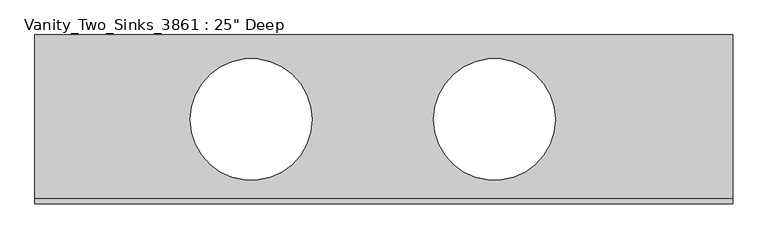
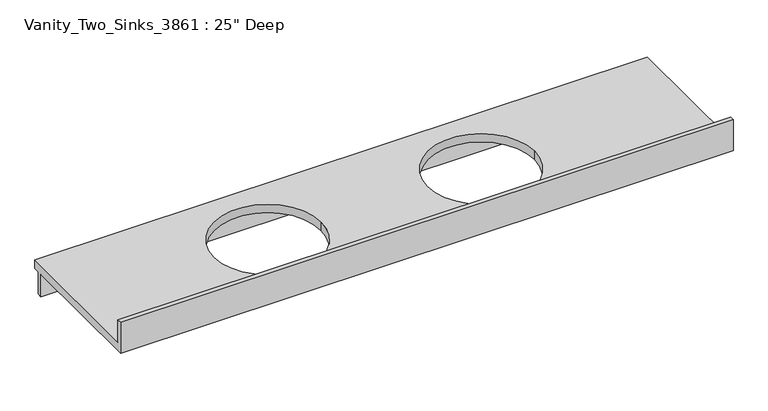
"""IFC4 building model written with IfcOpenShell, lengths in millimetres: furniture geometry."""

import ifcopenshell
import ifcopenshell.guid

model = None  # the IFC model being written
_history = None  # IfcOwnerHistory: only IFC2X3 demands one
_inside = {}  # id of a spatial element -> (the spatial element, [elements in it])
_under = {}  # id of a project, library or spatial element -> (it, [spatial elements below it])
_declared = {}  # id of a project -> (the project, [libraries it declares])
_typed = {}  # id of a type object -> (the type object, [elements of that type])
_made_of = {}  # id of a material, layer set ... -> (it, [elements and type objects made of it])


def new_model(schema):
    """Start an empty IFC model of exactly this schema.

    Asked for "IFC4X3", IfcOpenShell would pick the latest addendum, in which some entities
    have other attributes; the version numbers below select the first issue.
    IFC2X3 requires an IfcOwnerHistory on every rooted entity: one is made here for all.
    """
    global model, _history
    if schema == "IFC4X3":
        model = ifcopenshell.file(schema_version=(4, 3, 0, 0))
    else:
        model = ifcopenshell.file(schema=schema)
    _inside.clear()
    _under.clear()
    _declared.clear()
    _typed.clear()
    _made_of.clear()
    _history = None
    if model.schema == "IFC2X3":
        org = make("IfcOrganization", Name="unknown")
        user = make(
            "IfcPersonAndOrganization",
            ThePerson=make("IfcPerson", FamilyName="unknown"),
            TheOrganization=org,
        )
        app = make(
            "IfcApplication",
            ApplicationDeveloper=org,
            Version="unknown",
            ApplicationFullName="unknown",
            ApplicationIdentifier="unknown",
        )
        _history = make(
            "IfcOwnerHistory",
            OwningUser=user,
            OwningApplication=app,
            ChangeAction="ADDED",
            CreationDate=0,
        )
    return model


def make(cls, **values):
    """One entity of the class cls with the attributes given. An attribute that is None is left unset."""
    return model.create_entity(
        cls, **{name: value for name, value in values.items() if value is not None}
    )


def rooted(cls, **values):
    """An entity with a GlobalId (a new one), such as an element, a storey or a relation."""
    return make(cls, GlobalId=ifcopenshell.guid.new(), OwnerHistory=_history, **values)


def si_unit(unit_type, name, prefix=None):
    """IfcSIUnit, for example si_unit("LENGTHUNIT", "METRE", prefix="MILLI")."""
    return make("IfcSIUnit", UnitType=unit_type, Prefix=prefix, Name=name)


def assignment(units):
    """IfcUnitAssignment: the units of a project."""
    return None if units is None else make("IfcUnitAssignment", Units=units)


def point(xyz):
    """IfcCartesianPoint."""
    return None if xyz is None else make("IfcCartesianPoint", Coordinates=xyz)


def direction(xyz):
    """IfcDirection."""
    return None if xyz is None else make("IfcDirection", DirectionRatios=xyz)


def frame(location, z_axis=None, x_axis=None):
    """IfcAxis2Placement3D, a coordinate frame: its origin and axes. An axis left out is left unset."""
    return make(
        "IfcAxis2Placement3D",
        Location=point(location),
        Axis=direction(z_axis),
        RefDirection=direction(x_axis),
    )


def origin():
    """The frame at (0, 0, 0) with its axes left unset."""
    return frame((0.0, 0.0, 0.0))


def place(relative_to, where):
    """IfcLocalPlacement: puts the frame where relative to a parent placement (None: the world)."""
    return make(
        "IfcLocalPlacement", PlacementRelTo=relative_to, RelativePlacement=where
    )


def context(
    kind, dimensions, precision=None, world=None, true_north=None, identifier=None
):
    """IfcGeometricRepresentationContext, for example the 3D "Model" context."""
    return make(
        "IfcGeometricRepresentationContext",
        ContextIdentifier=identifier,
        ContextType=kind,
        CoordinateSpaceDimension=dimensions,
        Precision=precision,
        WorldCoordinateSystem=world,
        TrueNorth=true_north,
    )


def project(units=None, contexts=None):
    """IfcProject with its units and contexts."""
    return rooted(
        "IfcProject",
        Name="project",
        RepresentationContexts=contexts,
        UnitsInContext=assignment(units),
    )


def spatial(cls, under=None, at=None, **own):
    """A site, building, storey or space (cls), placed at a placement, below another one or the project."""
    s = rooted(cls, ObjectPlacement=at, **own)
    if under is not None:
        _under.setdefault(under.id(), (under, []))[1].append(s)
    return s


def polyline(points):
    """IfcPolyline through the points."""
    return make("IfcPolyline", Points=[point(p) for p in points])


def circle_curve(where, radius):
    """IfcCircle in the frame where."""
    return make("IfcCircle", Position=where, Radius=radius)


def shape(context_of_items, identifier, shape_type, items):
    """IfcShapeRepresentation: the items that make up one representation, for example the "Body"."""
    return make(
        "IfcShapeRepresentation",
        ContextOfItems=context_of_items,
        RepresentationIdentifier=identifier,
        RepresentationType=shape_type,
        Items=items,
    )


def source(mapping_origin, context_of_items, identifier, shape_type, items):
    """IfcRepresentationMap: a shape defined once, which mapped items show again and again."""
    return make(
        "IfcRepresentationMap",
        MappingOrigin=mapping_origin,
        MappedRepresentation=shape(context_of_items, identifier, shape_type, items),
    )


def transform(
    local_origin,
    x_axis=None,
    y_axis=None,
    z_axis=None,
    scale=None,
    scale2=None,
    scale3=None,
    uniform=True,
):
    """IfcCartesianTransformationOperator3D, or its non-uniform kind. x_axis, y_axis, z_axis: its Axis1, 2, 3."""
    if uniform:
        return make(
            "IfcCartesianTransformationOperator3D",
            Axis1=direction(x_axis),
            Axis2=direction(y_axis),
            LocalOrigin=point(local_origin),
            Scale=scale,
            Axis3=direction(z_axis),
        )
    return make(
        "IfcCartesianTransformationOperator3DnonUniform",
        Axis1=direction(x_axis),
        Axis2=direction(y_axis),
        LocalOrigin=point(local_origin),
        Scale=scale,
        Axis3=direction(z_axis),
        Scale2=scale2,
        Scale3=scale3,
    )


def mapped(mapping_source, mapping_target):
    """IfcMappedItem: shows the shape of a source again, moved by a transform."""
    return make(
        "IfcMappedItem", MappingSource=mapping_source, MappingTarget=mapping_target
    )


def made_of(thing, what):
    """Note that an element or type object is made of a material, layer set ...; save() writes the relation."""
    if what is not None:
        _made_of.setdefault(what.id(), (what, []))[1].append(thing)
    return thing


def element(
    cls,
    number,
    at=None,
    inside=None,
    cuts=None,
    type_object=None,
    material=None,
    context=None,
    identifier="Body",
    shape_type=None,
    held_by="IfcProductDefinitionShape",
    body=None,
    shapes=None,
    **own,
):
    """One element of the class cls, such as IfcWall. Its Tag is "e" and its number.

    at: its placement. inside: the storey or other place that contains it. cuts: it is an
    opening in that element (IfcRelVoidsElement). A single representation is given by context,
    identifier, shape_type and body (its items); several are given by shapes. held_by: the class
    of the entity that holds the representations. save() writes the other relations.
    """
    e = rooted(cls, Tag="e%d" % number, ObjectPlacement=at, **own)
    if body is not None:
        shapes = [shape(context, identifier, shape_type, body)]
    if shapes is not None:
        e.Representation = make(held_by, Representations=shapes)
    if inside is not None:
        _inside.setdefault(inside.id(), (inside, []))[1].append(e)
    if cuts is not None:
        rooted(
            "IfcRelVoidsElement", RelatingBuildingElement=cuts, RelatedOpeningElement=e
        )
    if type_object is not None:
        _typed.setdefault(type_object.id(), (type_object, []))[1].append(e)
    return made_of(e, material)


def aggregate(whole, parts):
    """IfcRelAggregates: a whole, such as a stair, and the parts it consists of."""
    return rooted("IfcRelAggregates", RelatingObject=whole, RelatedObjects=parts)


def save(model, path):
    """Write the relations noted so far, then the file.

    IfcRelAggregates (storeys below a building ...), IfcRelContainedInSpatialStructure (elements
    in a storey), IfcRelDefinesByType, IfcRelAssociatesMaterial and IfcRelDeclares: one each for
    every whole, place, type object, material and project.
    """
    for whole, parts in _under.values():
        aggregate(whole, parts)
    for where, things in _inside.values():
        rooted(
            "IfcRelContainedInSpatialStructure",
            RelatedElements=things,
            RelatingStructure=where,
        )
    for kind, things in _typed.values():
        rooted("IfcRelDefinesByType", RelatedObjects=things, RelatingType=kind)
    for what, things in _made_of.values():
        rooted("IfcRelAssociatesMaterial", RelatedObjects=things, RelatingMaterial=what)
    for by, libraries in _declared.values():
        rooted("IfcRelDeclares", RelatingContext=by, RelatedDefinitions=libraries)
    model.write(path)


def plane_surface(at):
    """IfcPlane: the flat surface through the origin of the frame at, square to its z axis."""
    return make("IfcPlane", Position=at)


def revolved_surface(curve, axis_point, axis_direction):
    """IfcSurfaceOfRevolution: the curve turned about the line through axis_point along axis_direction."""
    return make(
        "IfcSurfaceOfRevolution",
        SweptCurve=make("IfcArbitraryOpenProfileDef", ProfileType="CURVE", Curve=curve),
        AxisPosition=make("IfcAxis1Placement", Location=point(axis_point), Axis=direction(axis_direction)),
    )


def advanced_brep(points, edges, surfaces, faces):
    """IfcAdvancedBrep: a solid bounded by faces that lie on surfaces and meet in shared edges.

    An edge is (start, end): straight between two places in points (the first is 0);
    or (start, end, curve); or (start, end, curve, False) where it runs against its curve.
    A face is (place in surfaces, loops), or (place, loops, False) where it looks against
    its surface's normal. A loop lists edges by number (the first is 1), with a minus sign
    where the edge is run from its end to its start. The first loop is the outer one.
    """
    corners = [point(p) for p in points]
    vertices = [make("IfcVertexPoint", VertexGeometry=c) for c in corners]
    made = []
    for start, end, *more in edges:
        made.append(
            make(
                "IfcEdgeCurve",
                EdgeStart=vertices[start],
                EdgeEnd=vertices[end],
                EdgeGeometry=more[0] if more else make("IfcPolyline", Points=[corners[start], corners[end]]),
                SameSense=more[1] if len(more) > 1 else True,
            )
        )
    hull = []
    for where, loops, *sense in faces:
        bounds = []
        for j, loop in enumerate(loops):
            ring = [make("IfcOrientedEdge", EdgeElement=made[abs(k) - 1], Orientation=k > 0) for k in loop]
            bounds.append(
                make(
                    "IfcFaceOuterBound" if j == 0 else "IfcFaceBound",
                    Bound=make("IfcEdgeLoop", EdgeList=ring),
                    Orientation=True,
                )
            )
        hull.append(make("IfcAdvancedFace", Bounds=bounds, FaceSurface=surfaces[where], SameSense=sense[0] if sense else True))
    return make("IfcAdvancedBrep", Outer=make("IfcClosedShell", CfsFaces=hull))


def furniture_a1511c22(model_context):
    return source(origin(), model_context, "Body", "AdvancedBrep", [
        advanced_brep(
        [(-1327.4622951, 635.0, 863.6), (-1327.4622951, 19.05, 863.6), (1295.0877049, 19.05, 863.6), (1295.0877049, 635.0, 863.6), (628.3736357, 317.5, 863.6), (171.1736357, 317.5, 863.6), (-286.0263643, 317.5, 863.6), (-743.2263643, 317.5, 863.6), (1295.0877049, 635.0, 825.5), (1295.0877049, 609.6, 825.5), (-1327.4622951, 609.6, 825.5), (-1327.4622951, 635.0, 825.5), (-1327.4622951, 0.0, 825.5), (-1327.4622951, 590.55, 825.5), (1295.0877049, 590.55, 825.5), (1295.0877049, 0.0, 825.5), (171.1736357, 317.5, 825.5), (628.3736357, 317.5, 825.5), (-743.2263643, 317.5, 825.5), (-286.0263643, 317.5, 825.5), (1295.0877049, 0.0, 965.2), (-1327.4622951, 0.0, 965.2), (-1327.4622951, 609.6, 723.9), (-1327.4622951, 590.55, 723.9), (-1327.4622951, 19.05, 965.2), (1295.0877049, 19.05, 965.2), (1295.0877049, 590.55, 723.9), (1295.0877049, 609.6, 723.9)],
        [
            (0, 1),
            (1, 2),
            (2, 3),
            (3, 0),
            (4, 5, circle_curve(frame((399.7736357, 317.5, 863.6), z_axis=(0.0, 0.0, -1.0), x_axis=(1.0, 0.0, 0.0)), 228.6)),
            (5, 4, circle_curve(frame((399.7736357, 317.5, 863.6), z_axis=(0.0, 0.0, -1.0), x_axis=(1.0, 0.0, 0.0)), 228.6)),
            (6, 7, circle_curve(frame((-514.6263643, 317.5, 863.6), z_axis=(0.0, 0.0, -1.0), x_axis=(1.0, 0.0, 0.0)), 228.6)),
            (7, 6, circle_curve(frame((-514.6263643, 317.5, 863.6), z_axis=(0.0, 0.0, -1.0), x_axis=(1.0, 0.0, 0.0)), 228.6)),
            (8, 9),
            (9, 10),
            (10, 11),
            (11, 8),
            (12, 13),
            (13, 14),
            (14, 15),
            (15, 12),
            (16, 17, circle_curve(frame((399.7736357, 317.5, 825.5), z_axis=(0.0, 0.0, 1.0), x_axis=(1.0, 0.0, 0.0)), 228.6)),
            (17, 16, circle_curve(frame((399.7736357, 317.5, 825.5), z_axis=(0.0, 0.0, 1.0), x_axis=(1.0, 0.0, 0.0)), 228.6)),
            (18, 19, circle_curve(frame((-514.6263643, 317.5, 825.5), z_axis=(0.0, 0.0, 1.0), x_axis=(1.0, 0.0, 0.0)), 228.6)),
            (19, 18, circle_curve(frame((-514.6263643, 317.5, 825.5), z_axis=(0.0, 0.0, 1.0), x_axis=(1.0, 0.0, 0.0)), 228.6)),
            (15, 20),
            (20, 21),
            (21, 12),
            (10, 22),
            (22, 23),
            (23, 13),
            (21, 24),
            (24, 1),
            (0, 11),
            (3, 8),
            (2, 25),
            (25, 20),
            (14, 26),
            (26, 27),
            (27, 9),
            (5, 16),
            (17, 4),
            (25, 24),
            (7, 18),
            (19, 6),
            (26, 23),
            (22, 27),
        ],
        [
            plane_surface(frame((-1327.4622951, 0.0, 863.6), z_axis=(0.0, 0.0, 1.0), x_axis=(-1.0, 0.0, 0.0))),
            plane_surface(frame((-1327.4622951, 0.0, 825.5), z_axis=(0.0, 0.0, -1.0), x_axis=(1.0, 0.0, 0.0))),
            plane_surface(frame((1295.0877049, 0.0, 863.6), z_axis=(0.0, -1.0, 0.0), x_axis=(0.0, 0.0, -1.0))),
            plane_surface(frame((-1327.4622951, 0.0, 863.6), z_axis=(-1.0, 0.0, 0.0), x_axis=(0.0, 0.0, -1.0))),
            plane_surface(frame((-1327.4622951, 635.0, 863.6), z_axis=(0.0, 1.0, 0.0), x_axis=(0.0, 0.0, -1.0))),
            plane_surface(frame((1295.0877049, 635.0, 863.6), z_axis=(1.0, 0.0, 0.0), x_axis=(0.0, 0.0, -1.0))),
            revolved_surface(polyline([(628.3736357, 317.5, 863.6), (628.3736357, 317.5, 825.5)]), (399.7736357, 317.5, 825.5), (0.0, 0.0, 1.0)),
            plane_surface(frame((-1327.4622951, 0.0, 965.2), z_axis=(0.0, 0.0, 1.0), x_axis=(0.0, 1.0, 0.0))),
            plane_surface(frame((-1327.4622951, 19.05, 965.2), z_axis=(0.0, 1.0, 0.0), x_axis=(0.0, 0.0, -1.0))),
            revolved_surface(polyline([(-286.02636429999995, 317.5, 863.6), (-286.02636429999995, 317.5, 825.5)]), (-514.6263643, 317.5, 825.5), (0.0, 0.0, 1.0)),
            plane_surface(frame((-1327.4622951, 590.55, 723.9), z_axis=(0.0, 0.0, -1.0), x_axis=(1.0, 0.0, 0.0))),
            plane_surface(frame((1295.0877049, 590.55, 825.5), z_axis=(0.0, -1.0, 0.0), x_axis=(0.0, 0.0, -1.0))),
            plane_surface(frame((-1327.4622951, 609.6, 825.5), z_axis=(0.0, 1.0, 0.0), x_axis=(0.0, 0.0, -1.0))),
        ],
        [
            (0, [[1, 2, 3, 4], [5, 6], [7, 8]]),
            (1, [[9, 10, 11, 12]]),
            (1, [[13, 14, 15, 16], [17, 18], [19, 20]]),
            (2, [[21, 22, 23, -16]]),
            (3, [[-11, 24, 25, 26, -13, -23, 27, 28, -1, 29]]),
            (4, [[30, -12, -29, -4]]),
            (5, [[-3, 31, 32, -21, -15, 33, 34, 35, -9, -30]]),
            (6, [[-6, 36, -18, 37]]),
            (6, [[-17, -36, -5, -37]]),
            (7, [[-22, -32, 38, -27]]),
            (8, [[-31, -2, -28, -38]]),
            (9, [[-8, 39, -20, 40]]),
            (9, [[-19, -39, -7, -40]]),
            (10, [[41, -25, 42, -34]]),
            (11, [[-33, -14, -26, -41]]),
            (12, [[-24, -10, -35, -42]]),
        ],
    ),
    ])


if __name__ == "__main__":
    model = new_model("IFC4")
    model_context = context("Model", 3, world=origin())
    ifc_project = project(units=[si_unit("LENGTHUNIT", "METRE", prefix="MILLI")], contexts=[model_context])
    site = spatial("IfcSite", under=ifc_project)
    building = spatial("IfcBuilding", under=site)
    placement = place(None, origin())
    furniture_shape = furniture_a1511c22(model_context)
    element("IfcFurniture", 1, ObjectType="Vanity_Two_Sinks_3861 : 25\" Deep", at=placement, inside=building, context=model_context, shape_type="MappedRepresentation", body=[
        mapped(furniture_shape, transform((0.0, 0.0, 0.0), x_axis=(1.0, 0.0, 0.0), y_axis=(0.0, 1.0, 0.0), z_axis=(0.0, 0.0, 1.0))),
    ])
    save(model, "model.ifc")

# Revit data of these elements
# Type "Vanity_Two_Sinks_3861 : 25\" Deep"
#   Assembly Code = "C1030400"
#   Sink Location Right [instance default] = 1' - 6"
#   Counter Thickness = 0' - 1 1/2"
#   Depth = 2' - 1"
#   Height = 2' - 10"
#   Length [instance default] = 6' - 0"
#   Sink Location Left [instance default] = 1' - 6"
#   Sink to Back Wall = 0' - 4"
#   Sink Opening Width [instance default] = 1' - 5"
#   Counter Top = Casework - Vanity Top
#   Width = 0
# Element 1 (IfcFurniture, "Vanity_Two_Sinks_3861 : 25\" Deep")
#   Sink Location Right = 2' - 11.24859"
#   Length = 8' - 7 1/4"
#   Sink Location Left = 2' - 8.00141"
#   Materials on its faces: "Casework - Vanity Top"
# Materials
#   "Casework - Vanity Top": class "Unassigned", colour RGB 210 200 171, transparency 0, Comments = "Rendering appearance not upgraded "
